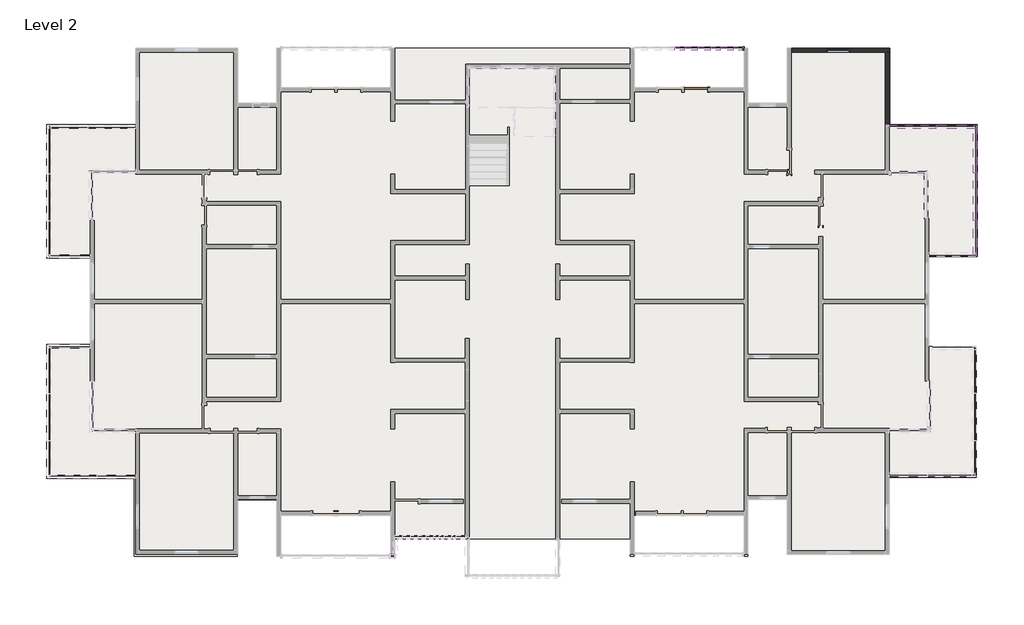
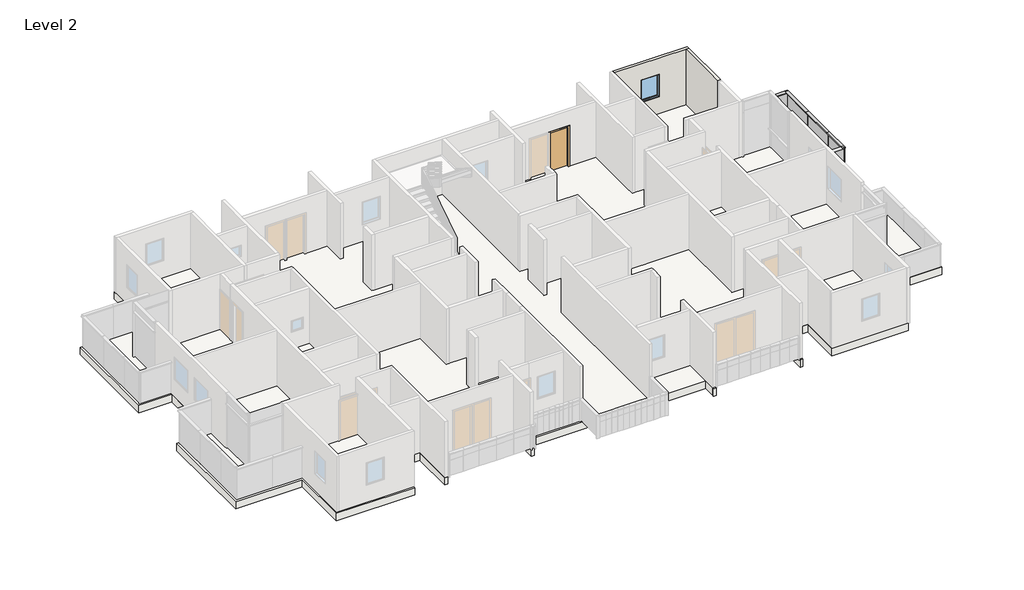
# One storey, part 5 of 7: 12 members, 11 plates, 2 walls, 1 door, 1 slab, 1 window.
"""IFC4 building model written with IfcOpenShell, lengths in millimetres."""

import ifcopenshell
import ifcopenshell.guid

model = None  # the IFC model being written
_history = None  # IfcOwnerHistory: only IFC2X3 demands one
_inside = {}  # id of a spatial element -> (the spatial element, [elements in it])
_under = {}  # id of a project, library or spatial element -> (it, [spatial elements below it])
_declared = {}  # id of a project -> (the project, [libraries it declares])
_typed = {}  # id of a type object -> (the type object, [elements of that type])
_made_of = {}  # id of a material, layer set ... -> (it, [elements and type objects made of it])


def new_model(schema):
    """Start an empty IFC model of exactly this schema.

    Asked for "IFC4X3", IfcOpenShell would pick the latest addendum, in which some entities
    have other attributes; the version numbers below select the first issue.
    IFC2X3 requires an IfcOwnerHistory on every rooted entity: one is made here for all.
    """
    global model, _history
    if schema == "IFC4X3":
        model = ifcopenshell.file(schema_version=(4, 3, 0, 0))
    else:
        model = ifcopenshell.file(schema=schema)
    _inside.clear()
    _under.clear()
    _declared.clear()
    _typed.clear()
    _made_of.clear()
    _history = None
    if model.schema == "IFC2X3":
        org = make("IfcOrganization", Name="unknown")
        user = make(
            "IfcPersonAndOrganization",
            ThePerson=make("IfcPerson", FamilyName="unknown"),
            TheOrganization=org,
        )
        app = make(
            "IfcApplication",
            ApplicationDeveloper=org,
            Version="unknown",
            ApplicationFullName="unknown",
            ApplicationIdentifier="unknown",
        )
        _history = make(
            "IfcOwnerHistory",
            OwningUser=user,
            OwningApplication=app,
            ChangeAction="ADDED",
            CreationDate=0,
        )
    return model


def make(cls, **values):
    """One entity of the class cls with the attributes given. An attribute that is None is left unset."""
    return model.create_entity(
        cls, **{name: value for name, value in values.items() if value is not None}
    )


def rooted(cls, **values):
    """An entity with a GlobalId (a new one), such as an element, a storey or a relation."""
    return make(cls, GlobalId=ifcopenshell.guid.new(), OwnerHistory=_history, **values)


def si_unit(unit_type, name, prefix=None):
    """IfcSIUnit, for example si_unit("LENGTHUNIT", "METRE", prefix="MILLI")."""
    return make("IfcSIUnit", UnitType=unit_type, Prefix=prefix, Name=name)


def assignment(units):
    """IfcUnitAssignment: the units of a project."""
    return None if units is None else make("IfcUnitAssignment", Units=units)


def point(xyz):
    """IfcCartesianPoint."""
    return None if xyz is None else make("IfcCartesianPoint", Coordinates=xyz)


def direction(xyz):
    """IfcDirection."""
    return None if xyz is None else make("IfcDirection", DirectionRatios=xyz)


def frame(location, z_axis=None, x_axis=None):
    """IfcAxis2Placement3D, a coordinate frame: its origin and axes. An axis left out is left unset."""
    return make(
        "IfcAxis2Placement3D",
        Location=point(location),
        Axis=direction(z_axis),
        RefDirection=direction(x_axis),
    )


def origin():
    """The frame at (0, 0, 0) with its axes left unset."""
    return frame((0.0, 0.0, 0.0))


def origin_with_axes():
    """The frame at (0, 0, 0) with the z axis (0, 0, 1) and the x axis (1, 0, 0) written out."""
    return frame((0.0, 0.0, 0.0), z_axis=(0.0, 0.0, 1.0), x_axis=(1.0, 0.0, 0.0))


def place(relative_to, where):
    """IfcLocalPlacement: puts the frame where relative to a parent placement (None: the world)."""
    return make(
        "IfcLocalPlacement", PlacementRelTo=relative_to, RelativePlacement=where
    )


def context(
    kind, dimensions, precision=None, world=None, true_north=None, identifier=None
):
    """IfcGeometricRepresentationContext, for example the 3D "Model" context."""
    return make(
        "IfcGeometricRepresentationContext",
        ContextIdentifier=identifier,
        ContextType=kind,
        CoordinateSpaceDimension=dimensions,
        Precision=precision,
        WorldCoordinateSystem=world,
        TrueNorth=true_north,
    )


def project(units=None, contexts=None):
    """IfcProject with its units and contexts."""
    return rooted(
        "IfcProject",
        Name="project",
        RepresentationContexts=contexts,
        UnitsInContext=assignment(units),
    )


def spatial(cls, under=None, at=None, **own):
    """A site, building, storey or space (cls), placed at a placement, below another one or the project."""
    s = rooted(cls, ObjectPlacement=at, **own)
    if under is not None:
        _under.setdefault(under.id(), (under, []))[1].append(s)
    return s


def polyline(points):
    """IfcPolyline through the points."""
    return make("IfcPolyline", Points=[point(p) for p in points])


def outline(outer, holes=None, kind="AREA"):
    """IfcArbitraryClosedProfileDef: a profile drawn as a closed curve; with holes, ...WithVoids."""
    if holes is None:
        return make("IfcArbitraryClosedProfileDef", ProfileType=kind, OuterCurve=outer)
    return make(
        "IfcArbitraryProfileDefWithVoids",
        ProfileType=kind,
        OuterCurve=outer,
        InnerCurves=holes,
    )


def extrude(swept, where, along, depth):
    """IfcExtrudedAreaSolid: the profile swept, set in the frame where, extruded along a direction by depth."""
    return make(
        "IfcExtrudedAreaSolid",
        SweptArea=swept,
        Position=where,
        ExtrudedDirection=direction(along),
        Depth=depth,
    )


def faces_of(points, faces, orient=None, outer=None):
    """IfcFace entities. A face is a list of loops; a loop is a list of indices into points, from 0.

    orient and outer hold one flag for each loop. By default every Orientation is true, the
    first loop of a face is its IfcFaceOuterBound and the others are IfcFaceBound.
    """
    made = []
    for i, loops in enumerate(faces):
        bounds = []
        for j, loop in enumerate(loops):
            is_outer = j == 0 if outer is None else outer[i][j]
            bounds.append(
                make(
                    "IfcFaceOuterBound" if is_outer else "IfcFaceBound",
                    Bound=make("IfcPolyLoop", Polygon=[points[k] for k in loop]),
                    Orientation=True if orient is None else orient[i][j],
                )
            )
        made.append(make("IfcFace", Bounds=bounds))
    return made


def faceted_brep(points, faces, orient=None, outer=None, voids=None):
    """IfcFacetedBrep: a solid bounded by flat faces; with voids (closed shells), ...WithVoids."""
    shared = [point(p) for p in points]
    hull = make("IfcClosedShell", CfsFaces=faces_of(shared, faces, orient, outer))
    if voids is None:
        return make("IfcFacetedBrep", Outer=hull)
    return make(
        "IfcFacetedBrepWithVoids",
        Outer=hull,
        Voids=[
            make(cls, CfsFaces=faces_of(shared, fs, o, b)) for cls, fs, o, b in voids
        ],
    )


def shape(context_of_items, identifier, shape_type, items):
    """IfcShapeRepresentation: the items that make up one representation, for example the "Body"."""
    return make(
        "IfcShapeRepresentation",
        ContextOfItems=context_of_items,
        RepresentationIdentifier=identifier,
        RepresentationType=shape_type,
        Items=items,
    )


def source(mapping_origin, context_of_items, identifier, shape_type, items):
    """IfcRepresentationMap: a shape defined once, which mapped items show again and again."""
    return make(
        "IfcRepresentationMap",
        MappingOrigin=mapping_origin,
        MappedRepresentation=shape(context_of_items, identifier, shape_type, items),
    )


def transform(
    local_origin,
    x_axis=None,
    y_axis=None,
    z_axis=None,
    scale=None,
    scale2=None,
    scale3=None,
    uniform=True,
):
    """IfcCartesianTransformationOperator3D, or its non-uniform kind. x_axis, y_axis, z_axis: its Axis1, 2, 3."""
    if uniform:
        return make(
            "IfcCartesianTransformationOperator3D",
            Axis1=direction(x_axis),
            Axis2=direction(y_axis),
            LocalOrigin=point(local_origin),
            Scale=scale,
            Axis3=direction(z_axis),
        )
    return make(
        "IfcCartesianTransformationOperator3DnonUniform",
        Axis1=direction(x_axis),
        Axis2=direction(y_axis),
        LocalOrigin=point(local_origin),
        Scale=scale,
        Axis3=direction(z_axis),
        Scale2=scale2,
        Scale3=scale3,
    )


def mapped(mapping_source, mapping_target):
    """IfcMappedItem: shows the shape of a source again, moved by a transform."""
    return make(
        "IfcMappedItem", MappingSource=mapping_source, MappingTarget=mapping_target
    )


def made_of(thing, what):
    """Note that an element or type object is made of a material, layer set ...; save() writes the relation."""
    if what is not None:
        _made_of.setdefault(what.id(), (what, []))[1].append(thing)
    return thing


def element(
    cls,
    number,
    at=None,
    inside=None,
    cuts=None,
    type_object=None,
    material=None,
    context=None,
    identifier="Body",
    shape_type=None,
    held_by="IfcProductDefinitionShape",
    body=None,
    shapes=None,
    **own,
):
    """One element of the class cls, such as IfcWall. Its Tag is "e" and its number.

    at: its placement. inside: the storey or other place that contains it. cuts: it is an
    opening in that element (IfcRelVoidsElement). A single representation is given by context,
    identifier, shape_type and body (its items); several are given by shapes. held_by: the class
    of the entity that holds the representations. save() writes the other relations.
    """
    e = rooted(cls, Tag="e%d" % number, ObjectPlacement=at, **own)
    if body is not None:
        shapes = [shape(context, identifier, shape_type, body)]
    if shapes is not None:
        e.Representation = make(held_by, Representations=shapes)
    if inside is not None:
        _inside.setdefault(inside.id(), (inside, []))[1].append(e)
    if cuts is not None:
        rooted(
            "IfcRelVoidsElement", RelatingBuildingElement=cuts, RelatedOpeningElement=e
        )
    if type_object is not None:
        _typed.setdefault(type_object.id(), (type_object, []))[1].append(e)
    return made_of(e, material)


def aggregate(whole, parts):
    """IfcRelAggregates: a whole, such as a stair, and the parts it consists of."""
    return rooted("IfcRelAggregates", RelatingObject=whole, RelatedObjects=parts)


def save(model, path):
    """Write the relations noted so far, then the file.

    IfcRelAggregates (storeys below a building ...), IfcRelContainedInSpatialStructure (elements
    in a storey), IfcRelDefinesByType, IfcRelAssociatesMaterial and IfcRelDeclares: one each for
    every whole, place, type object, material and project.
    """
    for whole, parts in _under.values():
        aggregate(whole, parts)
    for where, things in _inside.values():
        rooted(
            "IfcRelContainedInSpatialStructure",
            RelatedElements=things,
            RelatingStructure=where,
        )
    for kind, things in _typed.values():
        rooted("IfcRelDefinesByType", RelatedObjects=things, RelatingType=kind)
    for what, things in _made_of.values():
        rooted("IfcRelAssociatesMaterial", RelatedObjects=things, RelatingMaterial=what)
    for by, libraries in _declared.values():
        rooted("IfcRelDeclares", RelatingContext=by, RelatedDefinitions=libraries)
    model.write(path)


def m_single_flush_0915_x_2134mm_138fd904(model_context):
    return source(origin(), model_context, "Body", "SweptSolid", [
        extrude(outline(polyline([(2210.0, -533.5), (0.0, -533.5), (0.0, -457.5), (2134.0, -457.5), (2134.0, 457.5), (0.0, 457.5), (0.0, 533.5), (2210.0, 533.5), (2210.0, -533.5)])), frame((0.0, 75.0, 0.0), z_axis=(0.0, 1.0, 0.0), x_axis=(0.0, 0.0, 1.0)), (0.0, 0.0, 1.0), 25.0),
        extrude(outline(polyline([(2210.0, 533.5), (2210.0, -533.5), (0.0, -533.5), (0.0, -457.5), (2134.0, -457.5), (2134.0, 457.5), (0.0, 457.5), (0.0, 533.5), (2210.0, 533.5)])), frame((0.0, -100.0, 0.0), z_axis=(0.0, 1.0, 0.0), x_axis=(0.0, 0.0, 1.0)), (0.0, 0.0, 1.0), 25.0),
        extrude(outline(polyline([(457.5, 24.0), (-457.5, 24.0), (-457.5, 75.0), (457.5, 75.0), (457.5, 24.0)])), origin_with_axes(), (0.0, 0.0, 1.0), 2134.0),
    ])


def rectangular_mullion_50mm_x_150mm_42770ee2(model_context):
    return source(origin(), model_context, "Body", "SweptSolid", [
        extrude(outline(polyline([(0.0, 75.0), (0.0, -75.0), (-50.0, -75.0), (-50.0, 75.0), (0.0, 75.0)])), frame((0.0, 0.0, -1830.0000003), z_axis=(0.0, 0.0, 1.0), x_axis=(1.0, 0.0, 0.0)), (0.0, 0.0, 1.0), 1830.0000003),
    ])


def rectangular_mullion_50mm_x_150mm_aaee7d48(model_context):
    return source(origin(), model_context, "Body", "SweptSolid", [
        extrude(outline(polyline([(0.0, 75.0), (0.0, -75.0), (-50.0, -75.0), (-50.0, 75.0), (0.0, 75.0)])), frame((0.0, 0.0, -1830.0), z_axis=(0.0, 0.0, 1.0), x_axis=(1.0, 0.0, 0.0)), (0.0, 0.0, 1.0), 1830.0),
    ])


def rectangular_mullion_50mm_x_150mm_efa02866(model_context):
    return source(origin(), model_context, "Body", "SweptSolid", [
        extrude(outline(polyline([(0.0, 75.0), (0.0, -75.0), (-50.0, -75.0), (-50.0, 75.0), (0.0, 75.0)])), frame((0.0, 0.0, -1399.9999997), z_axis=(0.0, 0.0, 1.0), x_axis=(1.0, 0.0, 0.0)), (0.0, 0.0, 1.0), 1399.9999997),
    ])


def rectangular_mullion_50mm_x_150mm_d9f1e9e9(model_context):
    return source(origin(), model_context, "Body", "SweptSolid", [
        extrude(outline(polyline([(0.0, 75.0), (0.0, -75.0), (-50.0, -75.0), (-50.0, 75.0), (0.0, 75.0)])), frame((0.0, 0.0, -1565.8160321), z_axis=(0.0, 0.0, 1.0), x_axis=(1.0, 0.0, 0.0)), (0.0, 0.0, 1.0), 1565.8160321),
    ])


def rectangular_mullion_50mm_x_150mm_729c0cfc(model_context):
    return source(origin(), model_context, "Body", "SweptSolid", [
        extrude(outline(polyline([(0.0, 75.0), (0.0, -75.0), (-50.0, -75.0), (-50.0, 75.0), (0.0, 75.0)])), frame((0.0, 0.0, -1250.0), z_axis=(0.0, 0.0, 1.0), x_axis=(1.0, 0.0, 0.0)), (0.0, 0.0, 1.0), 1250.0),
    ])


def rectangular_mullion_50mm_x_150mm_b3666dbd(model_context):
    return source(origin(), model_context, "Body", "SweptSolid", [
        extrude(outline(polyline([(0.0, 75.0), (0.0, -75.0), (-50.0, -75.0), (-50.0, 75.0), (0.0, 75.0)])), frame((0.0, 0.0, -500.0), z_axis=(0.0, 0.0, 1.0), x_axis=(1.0, 0.0, 0.0)), (0.0, 0.0, 1.0), 500.0),
    ])


def rectangular_mullion_50mm_x_150mm_e11a3e7b(model_context):
    return source(origin(), model_context, "Body", "SweptSolid", [
        extrude(outline(polyline([(0.0, 75.0), (0.0, -75.0), (-50.0, -75.0), (-50.0, 75.0), (0.0, 75.0)])), frame((0.0, 0.0, -400.0), z_axis=(0.0, 0.0, 1.0), x_axis=(1.0, 0.0, 0.0)), (0.0, 0.0, 1.0), 400.0),
    ])


def rectangular_mullion_50mm_x_150mm_23485ade(model_context):
    return source(origin(), model_context, "Body", "SweptSolid", [
        extrude(outline(polyline([(0.0, 75.0), (0.0, -75.0), (-50.0, -75.0), (-50.0, 75.0), (0.0, 75.0)])), frame((0.0, 0.0, -350.0), z_axis=(0.0, 0.0, 1.0), x_axis=(1.0, 0.0, 0.0)), (0.0, 0.0, 1.0), 350.0),
    ])


def system_panel_glazed_09fbcc53(model_context):
    return source(origin(), model_context, "Body", "SweptSolid", [
        extrude(outline(polyline([(915.0000002, 24.5), (-915.0000002, 24.5), (-915.0000002, 49.5), (915.0000002, 49.5), (915.0000002, 24.5)])), origin_with_axes(), (0.0, 0.0, 1.0), 1200.0),
    ])


def system_panel_glazed_f4bbd109(model_context):
    return source(origin(), model_context, "Body", "SweptSolid", [
        extrude(outline(polyline([(910.8343113, 24.5), (-910.8343113, 24.5), (-910.8343113, 49.5), (910.8343113, 49.5), (910.8343113, 24.5)])), origin_with_axes(), (0.0, 0.0, 1.0), 1200.0),
    ])


def system_panel_glazed_42eec186(model_context):
    return source(origin(), model_context, "Body", "SweptSolid", [
        extrude(outline(polyline([(699.9999998, 24.5), (-699.9999998, 24.5), (-699.9999998, 49.5), (699.9999998, 49.5), (699.9999998, 24.5)])), origin_with_axes(), (0.0, 0.0, 1.0), 1200.0),
    ])


def system_panel_glazed_f2fc581d(model_context):
    return source(origin(), model_context, "Body", "SweptSolid", [
        extrude(outline(polyline([(782.9080161, 24.5), (-782.9080161, 24.5), (-782.9080161, 49.5), (782.9080161, 49.5), (782.9080161, 24.5)])), origin_with_axes(), (0.0, 0.0, 1.0), 1200.0),
    ])


def system_panel_glazed_346501af(model_context):
    return source(origin(), model_context, "Body", "SweptSolid", [
        extrude(outline(polyline([(250.0, 24.5), (-250.0, 24.5), (-250.0, 49.5), (250.0, 49.5), (250.0, 24.5)])), origin_with_axes(), (0.0, 0.0, 1.0), 1200.0),
    ])


def system_panel_glazed_3e660766(model_context):
    return source(origin(), model_context, "Body", "SweptSolid", [
        extrude(outline(polyline([(200.0, 24.5), (-200.0, 24.5), (-200.0, 49.5), (200.0, 49.5), (200.0, 24.5)])), origin_with_axes(), (0.0, 0.0, 1.0), 1200.0),
    ])


def system_panel_glazed_b0a6d7cd(model_context):
    return source(origin(), model_context, "Body", "SweptSolid", [
        extrude(outline(polyline([(175.0, 24.5), (-175.0, 24.5), (-175.0, 49.5), (175.0, 49.5), (175.0, 24.5)])), origin_with_axes(), (0.0, 0.0, 1.0), 1200.0),
    ])


def m_fixed_0915_x_1220mm_873aa0e2(model_context):
    return source(origin(), model_context, "Body", "SweptSolid", [
        extrude(outline(polyline([(-394.5, 53.0), (394.5, 53.0), (394.5, 41.0), (-394.5, 41.0), (-394.5, 53.0)])), frame((0.0, 0.0, 978.0), z_axis=(0.0, 0.0, 1.0), x_axis=(1.0, 0.0, 0.0)), (0.0, 0.0, 1.0), 1094.0),
        extrude(outline(polyline([(2116.0, -438.5), (934.0, -438.5), (934.0, 438.5), (2116.0, 438.5), (2116.0, -438.5)]), holes=[polyline([(2072.0, -394.5), (2072.0, 394.5), (978.0, 394.5), (978.0, -394.5), (2072.0, -394.5)])]), frame((0.0, 25.0, 0.0), z_axis=(0.0, 1.0, 0.0), x_axis=(0.0, 0.0, 1.0)), (0.0, 0.0, 1.0), 44.0),
        extrude(outline(polyline([(2135.0, -457.5), (915.0, -457.5), (915.0, 457.5), (2135.0, 457.5), (2135.0, -457.5)]), holes=[polyline([(2116.0, -438.5), (2116.0, 438.5), (934.0, 438.5), (934.0, -438.5), (2116.0, -438.5)])]), frame((0.0, 25.0, 0.0), z_axis=(0.0, 1.0, 0.0), x_axis=(0.0, 0.0, 1.0)), (0.0, 0.0, 1.0), 63.0),
        extrude(outline(polyline([(2135.0, -457.5), (915.0, -457.5), (915.0, 457.5), (2135.0, 457.5), (2135.0, -457.5)]), holes=[polyline([(2103.0, -425.5), (2103.0, 425.5), (947.0, 425.5), (947.0, -425.5), (2103.0, -425.5)])]), frame((0.0, -62.0, 0.0), z_axis=(0.0, 1.0, 0.0), x_axis=(0.0, 0.0, 1.0)), (0.0, 0.0, 1.0), 87.0),
    ])


model = new_model("IFC4")

# Units and contexts
model_context = context("Model", 3, world=origin())
ifc_project = project(units=[si_unit("LENGTHUNIT", "METRE", prefix="MILLI")], contexts=[model_context])

# Site, building, storey
site = spatial("IfcSite", under=ifc_project)
building = spatial("IfcBuilding", under=site)
storey = spatial("IfcBuildingStorey", under=building, Name="Level 2", Elevation=3500.0)

# Door
placement = place(None, origin())
m_single_flush_0915_x_2134mm_shape = m_single_flush_0915_x_2134mm_138fd904(model_context)
element("IfcDoor", 1, ObjectType="M_Single-Flush : 0915 x 2134mm", at=placement, inside=storey, context=model_context, shape_type="MappedRepresentation", body=[
    mapped(m_single_flush_0915_x_2134mm_shape, transform((6794.6515415, 8016.5690894, 3500.0), x_axis=(1.0, 0.0, 0.0), y_axis=(0.0, 1.0, 0.0), z_axis=(0.0, 0.0, 1.0))),
])

# Members
rectangular_mullion_50mm_x_150mm_shape = rectangular_mullion_50mm_x_150mm_42770ee2(model_context)
element("IfcMember", 2, ObjectType="Rectangular Mullion : 50mm x 150mm", at=placement, inside=storey, context=model_context, shape_type="MappedRepresentation", body=[
    mapped(rectangular_mullion_50mm_x_150mm_shape, transform((17635.0130284, 4788.3418163, 4750.0), x_axis=(0.0, 0.0, 1.0), y_axis=(-1.0, 0.0, 0.0), z_axis=(0.0, -1.0, 0.0))),
])
element("IfcMember", 3, ObjectType="Rectangular Mullion : 50mm x 150mm", at=placement, inside=storey, context=model_context, shape_type="MappedRepresentation", body=[
    mapped(rectangular_mullion_50mm_x_150mm_shape, transform((16129.1969963, 6568.8418166, 4750.0), x_axis=(0.0, 0.0, 1.0), y_axis=(0.0, -1.0, 0.0), z_axis=(1.0, 0.0, 0.0))),
])
rectangular_mullion_50mm_x_150mm_2_shape = rectangular_mullion_50mm_x_150mm_aaee7d48(model_context)
element("IfcMember", 4, ObjectType="Rectangular Mullion : 50mm x 150mm", at=placement, inside=storey, context=model_context, shape_type="MappedRepresentation", body=[
    mapped(rectangular_mullion_50mm_x_150mm_2_shape, transform((17635.0130284, 2958.3418163, 4750.0), x_axis=(0.0, 0.0, 1.0), y_axis=(-1.0, 0.0, 0.0), z_axis=(0.0, -1.0, 0.0))),
])
rectangular_mullion_50mm_x_150mm_3_shape = rectangular_mullion_50mm_x_150mm_efa02866(model_context)
element("IfcMember", 5, ObjectType="Rectangular Mullion : 50mm x 150mm", at=placement, inside=storey, context=model_context, shape_type="MappedRepresentation", body=[
    mapped(rectangular_mullion_50mm_x_150mm_3_shape, transform((17635.0130284, 1558.3418166, 4750.0), x_axis=(0.0, 0.0, 1.0), y_axis=(-1.0, 0.0, 0.0), z_axis=(0.0, -1.0, 0.0))),
])
rectangular_mullion_50mm_x_150mm_4_shape = rectangular_mullion_50mm_x_150mm_d9f1e9e9(model_context)
element("IfcMember", 6, ObjectType="Rectangular Mullion : 50mm x 150mm", at=placement, inside=storey, context=model_context, shape_type="MappedRepresentation", body=[
    mapped(rectangular_mullion_50mm_x_150mm_4_shape, transform((17695.0130284, 6568.8418166, 4750.0), x_axis=(0.0, 0.0, 1.0), y_axis=(0.0, -1.0, 0.0), z_axis=(1.0, 0.0, 0.0))),
])
rectangular_mullion_50mm_x_150mm_5_shape = rectangular_mullion_50mm_x_150mm_729c0cfc(model_context)
element("IfcMember", 7, ObjectType="Rectangular Mullion : 50mm x 150mm", at=placement, inside=storey, context=model_context, shape_type="MappedRepresentation", body=[
    mapped(rectangular_mullion_50mm_x_150mm_5_shape, transform((8667.3788142, 9614.2963621, 3500.0), x_axis=(1.0, 0.0, 0.0), y_axis=(0.0, -1.0, 0.0), z_axis=(0.0, 0.0, -1.0))),
])
rectangular_mullion_50mm_x_150mm_6_shape = rectangular_mullion_50mm_x_150mm_b3666dbd(model_context)
element("IfcMember", 8, ObjectType="Rectangular Mullion : 50mm x 150mm", at=placement, inside=storey, context=model_context, shape_type="MappedRepresentation", body=[
    mapped(rectangular_mullion_50mm_x_150mm_6_shape, transform((6867.3788142, 9614.2963621, 4750.0), x_axis=(0.0, 0.0, 1.0), y_axis=(0.0, -1.0, 0.0), z_axis=(1.0, 0.0, 0.0))),
])
element("IfcMember", 9, ObjectType="Rectangular Mullion : 50mm x 150mm", at=placement, inside=storey, context=model_context, shape_type="MappedRepresentation", body=[
    mapped(rectangular_mullion_50mm_x_150mm_6_shape, transform((7367.3788142, 9614.2963621, 4750.0), x_axis=(0.0, 0.0, 1.0), y_axis=(0.0, -1.0, 0.0), z_axis=(1.0, 0.0, 0.0))),
])
element("IfcMember", 10, ObjectType="Rectangular Mullion : 50mm x 150mm", at=placement, inside=storey, context=model_context, shape_type="MappedRepresentation", body=[
    mapped(rectangular_mullion_50mm_x_150mm_6_shape, transform((8267.3788142, 9614.2963621, 4750.0), x_axis=(0.0, 0.0, 1.0), y_axis=(0.0, -1.0, 0.0), z_axis=(1.0, 0.0, 0.0))),
])
rectangular_mullion_50mm_x_150mm_7_shape = rectangular_mullion_50mm_x_150mm_e11a3e7b(model_context)
element("IfcMember", 11, ObjectType="Rectangular Mullion : 50mm x 150mm", at=placement, inside=storey, context=model_context, shape_type="MappedRepresentation", body=[
    mapped(rectangular_mullion_50mm_x_150mm_7_shape, transform((6367.3788142, 9614.2963621, 4750.0), x_axis=(0.0, 0.0, 1.0), y_axis=(0.0, -1.0, 0.0), z_axis=(1.0, 0.0, 0.0))),
])
element("IfcMember", 12, ObjectType="Rectangular Mullion : 50mm x 150mm", at=placement, inside=storey, context=model_context, shape_type="MappedRepresentation", body=[
    mapped(rectangular_mullion_50mm_x_150mm_7_shape, transform((7767.3788142, 9614.2963621, 4750.0), x_axis=(0.0, 0.0, 1.0), y_axis=(0.0, -1.0, 0.0), z_axis=(1.0, 0.0, 0.0))),
])
rectangular_mullion_50mm_x_150mm_8_shape = rectangular_mullion_50mm_x_150mm_23485ade(model_context)
element("IfcMember", 13, ObjectType="Rectangular Mullion : 50mm x 150mm", at=placement, inside=storey, context=model_context, shape_type="MappedRepresentation", body=[
    mapped(rectangular_mullion_50mm_x_150mm_8_shape, transform((8617.3788142, 9614.2963621, 4750.0), x_axis=(0.0, 0.0, 1.0), y_axis=(0.0, -1.0, 0.0), z_axis=(1.0, 0.0, 0.0))),
])

# Plates
system_panel_glazed_shape = system_panel_glazed_09fbcc53(model_context)
element("IfcPlate", 14, ObjectType="System Panel : Glazed", at=placement, inside=storey, context=model_context, shape_type="MappedRepresentation", body=[
    mapped(system_panel_glazed_shape, transform((17635.0130284, 5703.3418165, 3500.0), x_axis=(0.0, -1.0, 0.0), y_axis=(1.0, 0.0, 0.0), z_axis=(0.0, 0.0, 1.0))),
])
element("IfcPlate", 15, ObjectType="System Panel : Glazed", at=placement, inside=storey, context=model_context, shape_type="MappedRepresentation", body=[
    mapped(system_panel_glazed_shape, transform((17635.0130284, 3873.3418163, 3500.0), x_axis=(0.0, -1.0, 0.0), y_axis=(1.0, 0.0, 0.0), z_axis=(0.0, 0.0, 1.0))),
])
system_panel_glazed_2_shape = system_panel_glazed_f4bbd109(model_context)
element("IfcPlate", 16, ObjectType="System Panel : Glazed", at=placement, inside=storey, context=model_context, shape_type="MappedRepresentation", body=[
    mapped(system_panel_glazed_2_shape, transform((16748.6787171, 1608.3418166, 3500.0), x_axis=(-1.0, 0.0, 0.0), y_axis=(0.0, -1.0, 0.0), z_axis=(0.0, 0.0, 1.0))),
])
system_panel_glazed_3_shape = system_panel_glazed_42eec186(model_context)
element("IfcPlate", 17, ObjectType="System Panel : Glazed", at=placement, inside=storey, context=model_context, shape_type="MappedRepresentation", body=[
    mapped(system_panel_glazed_3_shape, transform((17635.0130284, 2258.3418165, 3500.0), x_axis=(0.0, -1.0, 0.0), y_axis=(1.0, 0.0, 0.0), z_axis=(0.0, 0.0, 1.0))),
])
system_panel_glazed_4_shape = system_panel_glazed_f2fc581d(model_context)
element("IfcPlate", 18, ObjectType="System Panel : Glazed", at=placement, inside=storey, context=model_context, shape_type="MappedRepresentation", body=[
    mapped(system_panel_glazed_4_shape, transform((16912.1050124, 6568.8418166, 3500.0), x_axis=(1.0, 0.0, 0.0), y_axis=(0.0, 1.0, 0.0), z_axis=(0.0, 0.0, 1.0))),
])
system_panel_glazed_5_shape = system_panel_glazed_346501af(model_context)
element("IfcPlate", 19, ObjectType="System Panel : Glazed", at=placement, inside=storey, context=model_context, shape_type="MappedRepresentation", body=[
    mapped(system_panel_glazed_5_shape, transform((8017.3788142, 9614.2963621, 3500.0), x_axis=(1.0, 0.0, 0.0), y_axis=(0.0, 1.0, 0.0), z_axis=(0.0, 0.0, 1.0))),
])
element("IfcPlate", 20, ObjectType="System Panel : Glazed", at=placement, inside=storey, context=model_context, shape_type="MappedRepresentation", body=[
    mapped(system_panel_glazed_5_shape, transform((7117.3788142, 9614.2963621, 3500.0), x_axis=(1.0, 0.0, 0.0), y_axis=(0.0, 1.0, 0.0), z_axis=(0.0, 0.0, 1.0))),
])
element("IfcPlate", 21, ObjectType="System Panel : Glazed", at=placement, inside=storey, context=model_context, shape_type="MappedRepresentation", body=[
    mapped(system_panel_glazed_5_shape, transform((6617.3788142, 9614.2963621, 3500.0), x_axis=(1.0, 0.0, 0.0), y_axis=(0.0, 1.0, 0.0), z_axis=(0.0, 0.0, 1.0))),
])
system_panel_glazed_6_shape = system_panel_glazed_3e660766(model_context)
element("IfcPlate", 22, ObjectType="System Panel : Glazed", at=placement, inside=storey, context=model_context, shape_type="MappedRepresentation", body=[
    mapped(system_panel_glazed_6_shape, transform((7567.3788142, 9614.2963621, 3500.0), x_axis=(1.0, 0.0, 0.0), y_axis=(0.0, 1.0, 0.0), z_axis=(0.0, 0.0, 1.0))),
])
element("IfcPlate", 23, ObjectType="System Panel : Glazed", at=placement, inside=storey, context=model_context, shape_type="MappedRepresentation", body=[
    mapped(system_panel_glazed_6_shape, transform((6167.3788142, 9614.2963621, 3500.0), x_axis=(1.0, 0.0, 0.0), y_axis=(0.0, 1.0, 0.0), z_axis=(0.0, 0.0, 1.0))),
])
system_panel_glazed_7_shape = system_panel_glazed_b0a6d7cd(model_context)
element("IfcPlate", 24, ObjectType="System Panel : Glazed", at=placement, inside=storey, context=model_context, shape_type="MappedRepresentation", body=[
    mapped(system_panel_glazed_7_shape, transform((8442.3788142, 9614.2963621, 3500.0), x_axis=(1.0, 0.0, 0.0), y_axis=(0.0, 1.0, 0.0), z_axis=(0.0, 0.0, 1.0))),
])

# Slab
element("IfcSlab", 25, ObjectType="Generic Floor - 400mm", at=placement, inside=storey, context=model_context, shape_type="SweptSolid", body=[
    extrude(outline(polyline([(-10978.0757313, 7482.4781803), (-9455.3484585, 7482.4781803), (-9455.3484585, 9614.2963621), (-9305.3484585, 9614.2963621), (-9305.3484585, 8091.5690894), (-5039.4393676, 8091.5690894), (-5039.4393676, 9614.2963621), (4399.196996, 9614.2963621), (4399.196996, 8091.5690894), (8665.1060869, 8091.5690894), (8665.1060869, 9614.2963621), (8817.3788142, 9614.2963621), (8817.3788142, 7482.4781803), (10342.3783683, 7482.4781803), (10342.3783683, 9614.2963621), (14312.8444058, 9614.2963621), (14312.8444058, 6653.3418166), (17717.8444058, 6653.3418166), (17717.8444058, 1533.3418166), (15837.8444058, 1533.3418166), (15837.8444058, -1946.1581834), (17677.8444058, -1946.1581834), (17677.8444058, -7028.8854561), (14240.1060869, -7028.8854561), (14240.1060869, -10028.8854561), (10340.1060869, -10028.8854561), (10340.1060869, -7894.794547), (8815.1060869, -7894.794547), (8815.1060869, -10106.1581834), (8665.1060869, -10106.1581834), (8665.1060869, -8506.1581834), (4401.4697233, -8506.1581834), (4401.4697233, -10106.1581834), (4251.4697233, -10106.1581834), (4251.4697233, -10028.8854561), (4251.4697233, -9417.5218198), (-4887.1666404, -9417.5218198), (-4887.1666404, -10006.7413208), (-4887.1666404, -10106.1581834), (-5039.4393676, -10106.1581834), (-5039.4393676, -8503.8854561), (-9303.0757313, -8503.8854561), (-9303.0757313, -10106.1581834), (-9453.0757313, -10106.1581834), (-9453.0757313, -7906.1581834), (-10989.3512663, -7906.1581834), (-10989.3512663, -10106.1581834), (-14989.3512663, -10106.1581834), (-14989.3512663, -7083.4309107), (-18389.3512663, -7083.4309107), (-18389.3512663, -1883.4309107), (-16697.1666404, -1883.4309107), (-16697.1666404, 1474.2963621), (-18377.1666404, 1474.2963621), (-18377.1666404, 6654.2963621), (-14937.1666404, 6654.2963621), (-14937.1666404, 9614.2963621), (-10978.0757313, 9614.2963621), (-10978.0757313, 7482.4781803)])), frame((0.0, 0.0, 3100.0), z_axis=(0.0, 0.0, 1.0), x_axis=(1.0, 0.0, 0.0)), (0.0, 0.0, 1.0), 400.0),
])

# Walls
element("IfcWall", 26, ObjectType="wal 150", at=placement, inside=storey, context=model_context, shape_type="Brep", body=[
    faceted_brep([(10492.3783683, 9464.2963621, 3500.0), (14149.196996, 9464.2963621, 3500.0), (14299.196996, 9464.2963621, 3500.0), (14299.196996, 9464.2963621, 6500.0), (14149.196996, 9464.2963621, 6500.0), (10492.3783683, 9464.2963621, 6500.0), (11863.2876822, 9464.2963621, 4415.0), (11863.2876822, 9464.2963621, 5635.0), (12778.2876822, 9464.2963621, 5635.0), (12778.2876822, 9464.2963621, 4415.0), (10492.3783683, 9614.2963621, 3500.0), (10492.3783683, 9614.2963621, 6500.0), (14299.196996, 9614.2963621, 6500.0), (14299.196996, 9614.2963621, 3500.0), (11863.2876822, 9614.2963621, 4415.0), (12778.2876822, 9614.2963621, 4415.0), (12778.2876822, 9614.2963621, 5635.0), (11863.2876822, 9614.2963621, 5635.0)], [[[0, 1, 2, 3, 4, 5], [6, 7, 8, 9]], [[10, 11, 12, 13], [14, 15, 16, 17]], [[2, 1, 0, 10, 13]], [[5, 4, 3, 12, 11]], [[7, 6, 14, 17]], [[8, 7, 17, 16]], [[9, 8, 16, 15]], [[6, 9, 15, 14]], [[0, 5, 11, 10]], [[3, 2, 13, 12]]]),
])
element("IfcWall", 27, ObjectType="wal 150", at=placement, inside=storey, context=model_context, shape_type="SweptSolid", body=[
    extrude(outline(polyline([(14149.196996, 6668.8418166), (14149.196996, 9464.2963621), (14299.196996, 9464.2963621), (14299.196996, 6668.8418166), (14149.196996, 6668.8418166)])), frame((0.0, 0.0, 3500.0), z_axis=(0.0, 0.0, 1.0), x_axis=(1.0, 0.0, 0.0)), (0.0, 0.0, 1.0), 3000.0),
])

# Window
m_fixed_0915_x_1220mm_shape = m_fixed_0915_x_1220mm_873aa0e2(model_context)
element("IfcWindow", 28, ObjectType="M_Fixed : 1.80 to 1.20 w2", at=placement, inside=storey, context=model_context, shape_type="MappedRepresentation", body=[
    mapped(m_fixed_0915_x_1220mm_shape, transform((12320.7876822, 9526.2963621, 3500.0), x_axis=(1.0, 0.0, 0.0), y_axis=(0.0, 1.0, 0.0), z_axis=(0.0, 0.0, 1.0))),
])

save(model, "model.ifc")

# Revit data of these elements
# Project information
#   Project Issue Date = "Issue Date"
#   Project Status = "Project  Status"
#   Client Name = "Owner"
#   Project Address = "## Street\nCity, State  Zip"
#   Project Name = "Project Name"
#   Project Number = "Project  Number"
# Type "M_Single-Flush : 0915 x 2134mm"
#   Type Mark = "15"
#   Thickness = 0.051 m
#   Height = 2.134 m
#   Trim Projection Ext = 0.025 m
#   Trim Projection Int = 0.025 m
#   Trim Width = 0.076 m
#   Width = 0.915 m
#   Door Material = Door - Panel
#   Frame Material = Door - Frame
#   Function = (empty or 0)
#   Wall Closure = (empty or 0)
# Type "Rectangular Mullion : 50mm x 150mm"
#   built-in parameter 1007304 = 0.492126 (stored number, unit not read)
#   built-in parameter 1007301 = 0.082021 (stored number, unit not read)
#   built-in parameter 1007300 = 0.082021 (stored number, unit not read)
# Type "Generic Floor - 400mm"
#   Function = 0
#   Layers, outside or top first: 0.4 m no material (function 1)
# Type "wal 150"
#   Layers, outside or top first: 0.15 m no material (function 1)
# Type "M_Fixed : 1.80 to 1.20 w2"
#   Type Mark = "19"
#   Height = 1.22 m
#   Default Sill Height = 0.915 m
#   Width = 0.915 m
#   Window Inset = 0.019 m
#   Frame Exterior Material = Sash
#   Frame Interior Material = Sash
#   Glass Pane Material = Glass
#   Sash = Sash
#   Wall Closure = (empty or 0)
# Element 1 (IfcDoor, "M_Single-Flush : 0915 x 2134mm")
#   Phase Created = New Construction
#   Materials on its faces: "Door - Frame", "Door - Panel"
# Elements 2, 3, 4, 5, 6, 7, 8, 9, 10, 11, 12, 13 (IfcMember, "Rectangular Mullion : 50mm x 150mm")
#   Phase Created = New Construction
#   Materials on its faces: "Aluminum"
# Elements 14, 15, 16, 17, 18, 19, 20, 21, 22, 23, 24 (IfcPlate, "System Panel : Glazed")
#   Phase Created = New Construction
#   Materials on its faces: "Glass"
# Element 25 (IfcSlab, "Generic Floor - 400mm")
#   built-in parameter 1001955 = 3.14159 (stored number, unit not read)
#   Height Offset From Level = 0 m
#   Phase Created = New Construction
#   Materials on its faces: "Default Roof", "Door - Frame", "Ceiling Tile 600 x 1200", "Oak Flooring"
# Element 26 (IfcWall, "wal 150")
#   Top Offset = 0 m
#   Base Offset = 0 m
#   Unconnected Height = 3 m
#   wall height = 3 m
#   Phase Created = New Construction
#   Base Constraint = Level 2
#   Materials on its faces: "Default Wall", "Ceiling Tile 600 x 600", "Ceiling Tile 600 x 1200"
# Element 27 (IfcWall, "wal 150")
#   Top Offset = 0 m
#   Base Offset = 0 m
#   Unconnected Height = 3 m
#   wall height = 3 m
#   Phase Created = New Construction
#   Base Constraint = Level 2
#   Materials on its faces: "Default Wall", "Ceiling Tile 600 x 1200"
# Element 28 (IfcWindow, "M_Fixed : 1.80 to 1.20 w2")
#   Mark = "14"
#   Phase Created = New Construction
#   Materials on its faces: "Sash", "Glass"
# Materials
#   "Door - Panel": class "Wood", colour RGB 114 82 51, transparency 0
#   "Door - Frame": class "Miscellaneous", colour RGB 255 0 128, transparency 0, Cost = 0
#   "Sash": class "Wood", colour RGB 136 99 55, transparency 0
#   "Glass": class "Glass", colour RGB 218 227 224, transparency 0.85, Description = "Soda Lime Glass", Cost = 0
#   "Aluminum": class "Metal", colour RGB 244 244 244, transparency 0, Description = "Aluminum 6061", Cost = 0
#   "Default Roof": class "Miscellaneous", colour RGB 80 80 80, transparency 0
#   "Ceiling Tile 600 x 1200": class "Generic", colour RGB 179 178 175, transparency 0, Description = "Acoustic ceiling tile", Cost = 0
#   "Oak Flooring": class "Wood", colour RGB 216 169 114, transparency 0, Description = "Quercus Rubra", Cost = 0
#   "Default Wall": class "Miscellaneous", colour RGB 80 80 80, transparency 0
#   "Ceiling Tile 600 x 600": class "Generic", colour RGB 180 179 177, transparency 0, Description = "Acoustic ceiling tile", Cost = 0
